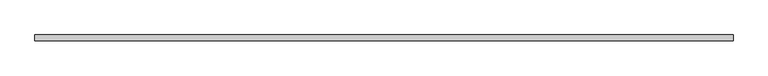
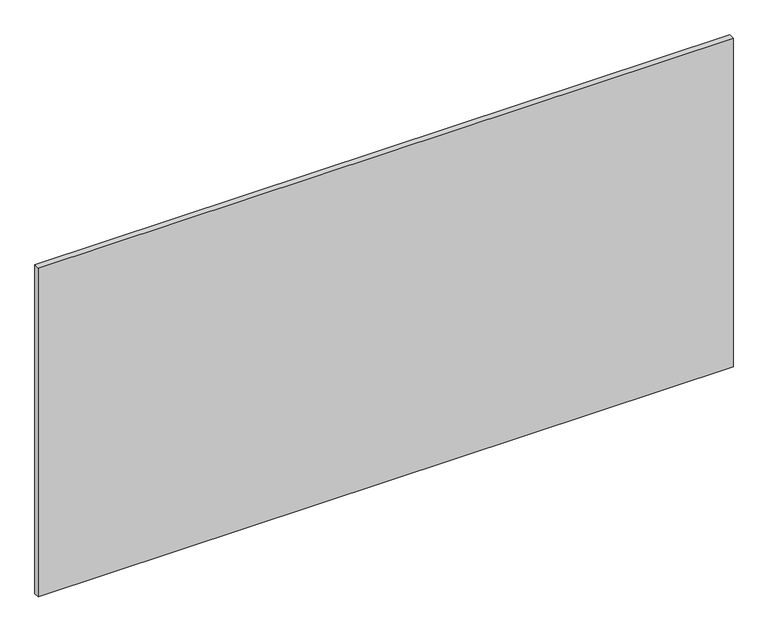
"""IFC4 building model written with IfcOpenShell, lengths in millimetres: proxy geometry, Vertical furring:Vertical furring:3:Vertical furring:3 : Vertical furring:Vertical furring:300288:353074:Vertical furring:3:Vertical furring:3 : Vertical furring:Vertical furring:300288:353074 : Vertical furring:Vertical furring:3:Vertical furring:3 : Vertical furring:Vertical furring:300288:353074:3 : Vertical furring:Vertical furring:3:Vertical furring:3 : Vertical furring:Vertical furring:300288:353074:Vertical furring:3:Vertical furring:3 : Vertical furring:Vertical furring:300288:353074 : Vertical furring:Vertical furring:3:Vertical furring:3 : Vertical furring:Vertical furring:300288:353074:301917."""

from ifc_helpers import new_model, si_unit, frame, origin, place, context, project, spatial, polyline, outline, extrude, source, transform, mapped, element, save


def generic_models_d4f18349(model_context):
    return source(origin(), model_context, "Body", "SweptSolid", [
        extrude(outline(polyline([(593738.0867239, -579018.1880937), (596176.4867239, -579018.1880937), (596176.4867239, -579038.7913841), (593738.0867239, -579038.7913841), (593738.0867239, -579018.1880937)])), frame((0.0, 0.0, 2451.1), z_axis=(0.0, 0.0, 1.0), x_axis=(1.0, 0.0, 0.0)), (0.0, 0.0, 1.0), 1219.2),
    ])


if __name__ == "__main__":
    model = new_model("IFC4")
    model_context = context("Model", 3, world=origin())
    ifc_project = project(units=[si_unit("LENGTHUNIT", "METRE", prefix="MILLI")], contexts=[model_context])
    site = spatial("IfcSite", under=ifc_project)
    building = spatial("IfcBuilding", under=site)
    placement = place(None, origin())
    generic_models_shape = generic_models_d4f18349(model_context)
    element("IfcBuildingElementProxy", 1, Name="Vertical furring:Vertical furring:3:Vertical furring:3 : Vertical furring:Vertical furring:300288:353074:Vertical furring:3:Vertical furring:3 : Vertical furring:Vertical furring:300288:353074 : Vertical furring:Vertical furring:3:Vertical furring:3 : Vertical furring:Vertical furring:300288:353074:3 : Vertical furring:Vertical furring:3:Vertical furring:3 : Vertical furring:Vertical furring:300288:353074:Vertical furring:3:Vertical furring:3 : Vertical furring:Vertical furring:300288:353074 : Vertical furring:Vertical furring:3:Vertical furring:3 : Vertical furring:Vertical furring:300288:353074:301917", ObjectType="Vertical furring:Vertical furring:3:Vertical furring:3 : Vertical furring:Vertical furring:300288:353074:Vertical furring:3:Vertical furring:3 : Vertical furring:Vertical furring:300288:353074 : Vertical furring:Vertical furring:3:Vertical furring:3 : Vertical furring:Vertical furring:300288:353074:3 : Vertical furring:Vertical furring:3:Vertical furring:3 : Vertical furring:Vertical furring:300288:353074:Vertical furring:3:Vertical furring:3 : Vertical furring:Vertical furring:300288:353074 : Vertical furring:Vertical furring:3:Vertical furring:3 : Vertical furring:Vertical furring:300288:353074:301917", at=placement, inside=building, context=model_context, shape_type="MappedRepresentation", body=[
        mapped(generic_models_shape, transform((0.0, 0.0, 0.0), x_axis=(1.0, 0.0, 0.0), y_axis=(0.0, 1.0, 0.0), z_axis=(0.0, 0.0, 1.0))),
    ])
    save(model, "model.ifc")

# Revit data of these elements
# Type "Vertical furring:Vertical furring:3:Vertical furring:3 : Vertical furring:Vertical furring:300288:353074:Vertical furring:3:Vertical furring:3 : Vertical furring:Vertical furring:300288:353074 : Vertical furring:Vertical furring:3:Vertical furring:3 : Vertical furring:Vertical furring:300288:353074:3 : Vertical furring:Vertical furring:3:Vertical furring:3 : Vertical furring:Vertical furring:300288:353074:Vertical furring:3:Vertical furring:3 : Vertical furring:Vertical furring:300288:353074 : Vertical furring:Vertical furring:3:Vertical furring:3 : Vertical furring:Vertical furring:300288:353074:301917"
#   NameOverride = "Vertical furring:Vertical furring:3:Vertical furring:3 : Vertical furring:Vertical furring:300288:353074:Vertical furring:3:Vertical furring:3 : Vertical furring:Vertical furring:300288:353074 : Vertical furring:Vertical furring:3:Vertical furring:3 : Vertical furring:Vertical furring:300288:353074:301917"
#   ObjectTypeOverride = "Vertical furring:3:Vertical furring:3 : Vertical furring:Vertical furring:300288:353074 : Vertical furring:Vertical furring:3:Vertical furring:3 : Vertical furring:Vertical furring:300288:353074"
#   Reference = "Vertical furring"
#   Tag = "301917"
# Element 1 (IfcBuildingElementProxy, "Vertical furring:Vertical furring:3:Vertical furring:3 : Vertical furring:Vertical furring:300288:353074:Vertical furring:3:Vertical furring:3 : Vertical furring:Vertical furring:300288:353074 : Vertical furring:Vertical furring:3:Vertical furring:3 : Vertical furring:Vertical furring:300288:353074:3 : Vertical furring:Vertical furring:3:Vertical furring:3 : Vertical furring:Vertical furring:300288:353074:Vertical furring:3:Vertical furring:3 : Vertical furring:Vertical furring:300288:353074 : Vertical furring:Vertical furring:3:Vertical furring:3 : Vertical furring:Vertical furring:300288:353074:301917")
#   Materials on its faces: "1\" MINERAL WOOL BOARD INSULATION"
# Materials
#   "1\" MINERAL WOOL BOARD INSULATION": class "Unassigned", colour RGB 205 188 106, transparency 0, Cost = 0
